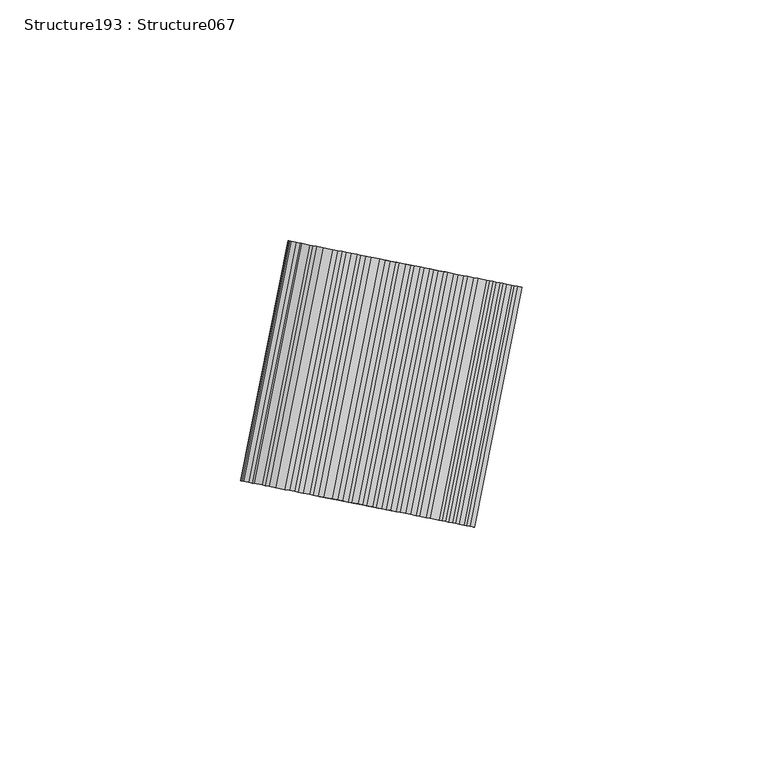
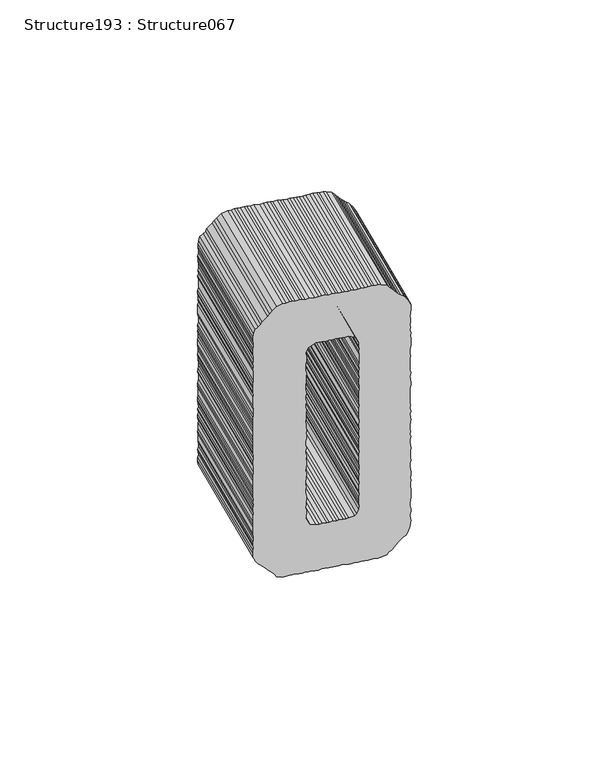
"""IFC4 building model written with IfcOpenShell, lengths in millimetres: proxy geometry, Structure193 : Structure067."""

from ifc_helpers import new_model, si_unit, frame, origin, place, context, project, spatial, polyline, outline, extrude, source, transform, mapped, element, save


def structure193_structure067_310a77a5(model_context):
    return source(origin(), model_context, "Body", "SweptSolid", [
        extrude(outline(polyline([(1.9860445, 0.0), (2.6789094, -0.7882832), (3.8239592, -1.2173664), (5.3807844, -2.3653471), (6.3497852, -3.2236496), (7.0882408, -3.6107772), (8.0066377, -4.2175769), (9.1528806, -4.65259), (9.8415639, -5.445344), (10.8594989, -7.2214925), (11.1707558, -8.0920017), (11.5266802, -9.2097639), (11.5546014, -9.9997252), (11.6286641, -11.0442649), (12.1416474, -12.266168), (12.3476425, -13.2899692), (12.2954284, -14.3581017), (12.5003006, -15.3763217), (12.8104345, -16.2412497), (13.1408113, -17.2320396), (13.7306521, -20.1635644), (13.8103704, -21.2109584), (14.040369, -22.3540577), (14.3966443, -23.4735641), (14.4256886, -24.2691066), (14.781613, -25.3868688), (14.9872571, -26.4089259), (15.0395329, -27.3199294), (15.139845, -28.4949295), (15.3454892, -29.5169867), (15.7807769, -30.3527405), (15.8859726, -31.526758), (16.3216154, -33.6919144), (16.6775398, -34.8096767), (16.7321316, -35.7321914), (16.8312506, -36.9012615), (17.0114174, -37.7966951), (17.4985021, -38.8898819), (17.4210914, -39.8327863), (17.7826715, -40.9534029), (17.8049371, -41.7405098), (18.0616063, -43.0161625), (18.7284366, -45.0026899), (18.7567089, -45.7943953), (18.8558279, -46.9634655), (19.2919578, -47.8034053), (19.2408667, -48.877119), (19.6016747, -49.9938986), (19.6764393, -51.0419265), (20.7011507, -56.1347704), (21.1636003, -57.1055196), (21.3935287, -58.2482701), (21.4218009, -59.0399755), (21.5221131, -60.2149756), (22.0339734, -61.4312976), (21.9577558, -62.3801319), (22.7775952, -66.454756), (23.138333, -67.5711868), (23.2132379, -68.6199123), (23.4180399, -69.6377835), (24.0334943, -71.368971), (24.4953163, -73.664239), (24.5743328, -74.7081449), (24.8784601, -75.5684743), (24.8021724, -76.5169599), (25.1629804, -77.6337395), (25.2126185, -78.556888), (25.5734967, -79.6740165), (25.7528914, -80.5656131), (25.8276559, -81.6136409), (26.5443883, -83.8481827), (26.9297079, -85.7632317), (26.371283, -87.5984982), (25.7853557, -88.6440823), (25.4039476, -89.3802981), (24.5409722, -90.351328), (23.9028991, -91.1395494), (23.397037, -91.9066133), (22.8107609, -92.9522675), (22.304197, -93.7158431), (21.6937749, -94.6396873), (21.2071753, -95.5295438), (19.5530517, -96.5280079), (18.6869304, -96.8322118), (17.412673, -97.0886002), (16.6774334, -97.3686475), (15.5294505, -97.5996287), (14.4863807, -97.6773882), (13.338049, -97.9084396), (12.4216748, -97.9628847), (11.2782267, -98.1929535), (10.4068731, -98.4982102), (9.4904989, -98.5526553), (8.3721773, -98.9076035), (7.5817289, -98.9367116), (6.3074714, -99.1931), (5.5669273, -99.472037), (4.5753013, -99.8036708), (3.2503698, -99.8082076), (2.535722, -100.2140467), (1.3922738, -100.4441155), (0.3443204, -100.5228576), (-0.8287889, -100.6289594), (-2.5564243, -101.2386178), (-3.7550812, -101.2177474), (-4.7219295, -101.6743307), (-5.4872513, -101.8283182), (-6.7870564, -101.9577344), (-7.7790312, -102.2894384), (-8.544353, -102.4434258), (-9.6125495, -102.396306), (-10.6349554, -102.6020203), (-12.672446, -102.3463317), (-14.3292984, -101.3524044), (-15.2483972, -100.7421164), (-16.0409385, -100.1096308), (-18.0013673, -98.911108), (-18.5634229, -98.0965052), (-19.4562021, -97.6170265), (-20.6279926, -97.0550411), (-21.3186987, -95.6010422), (-21.674623, -94.48328), (-21.9046216, -93.3401807), (-21.9842698, -92.2931354), (-22.1635943, -91.4018877), (-22.626465, -90.4290457), (-22.6749099, -89.5118271), (-22.8794311, -88.4953512), (-22.9583774, -87.4517943), (-23.189499, -86.3031137), (-23.5461954, -85.1815144), (-23.6250715, -84.1383062), (-24.0611312, -83.2987152), (-24.0101104, -82.2246527), (-24.650555, -79.0416252), (-25.0854918, -78.2076154), (-25.3166134, -77.0589349), (-25.340002, -76.2662469), (-25.59625, -74.9926871), (-25.6497189, -74.0757535), (-26.0857786, -73.2361625), (-26.7262233, -70.0531351), (-26.7258063, -68.7275697), (-27.1099328, -66.8184508), (-27.5468347, -65.974674), (-27.6715013, -64.6786316), (-27.9565789, -63.9382341), (-28.0314137, -62.8898573), (-28.2358647, -61.8737304), (-28.5727394, -60.8759), (-28.9808693, -58.847483), (-29.0556339, -57.7994551), (-29.2605761, -56.7808864), (-29.6476336, -55.5336463), (-29.6973419, -54.6101489), (-29.9017929, -53.5940218), (-29.9818622, -52.5448836), (-30.1856113, -51.5322449), (-30.5422375, -50.4109944), (-30.879042, -49.4135129), (-30.8005084, -48.4761896), (-31.1855472, -46.5625361), (-31.6722108, -45.4714423), (-31.8527285, -44.5742647), (-31.9519177, -43.4048457), (-32.4130378, -41.1130659), (-32.7231718, -40.2481378), (-32.9280439, -39.2299179), (-33.0028786, -38.1815412), (-33.1080744, -37.0075237), (-33.5430111, -36.1735138), (-33.5173975, -34.9731767), (-33.9279798, -34.2602091), (-34.1336239, -33.2381521), (-34.1072383, -32.041652), (-34.4125587, -31.1753925), (-34.8481313, -29.010585), (-35.1571423, -28.1512381), (-35.2323279, -27.1011173), (-35.6930972, -24.8110817), (-35.7731664, -23.7619435), (-35.952491, -22.8706958), (-36.4137474, -21.9058766), (-36.4622624, -20.9883093), (-36.5419808, -19.9409152), (-37.0035881, -18.9743519), (-37.2335867, -17.8312526), (-37.3338989, -16.6562525), (-36.8766221, -14.9712725), (-36.4462117, -13.8274074), (-35.8096105, -13.033675), (-35.3026977, -12.2700292), (-34.6660964, -11.4762968), (-33.9527013, -10.4112356), (-33.4723868, -9.5171994), (-32.3486946, -7.8360522), (-31.8935768, -6.8167879), (-30.2394531, -5.8183238), (-29.0648018, -5.7180817), (-28.022153, -5.6382292), (-27.1560318, -5.3340255), (-26.2393088, -5.27951), (-25.1209872, -4.924562), (-24.2248559, -4.7442549), (-22.925472, -4.6127457), (-22.1901602, -4.3348616), (-21.016702, -4.2286895), (-20.1765516, -3.7936062), (-19.1593781, -3.5889446), (-18.0855261, -3.6389189), (-17.1942784, -3.4595944), (-16.0759568, -3.1046463), (-13.0139715, -2.4885561), (-11.9762063, -2.4096862), (-10.9541492, -2.2040421), (-9.9880731, -1.7436217), (-9.0968253, -1.5642972), (-8.1740256, -1.5147293), (-7.0568972, -1.1538512), (-5.8574682, -1.1785586), (-4.9909981, -0.8742846), (-3.9734759, -0.6695529), (-2.8003666, -0.5634509), (-1.7828442, -0.3587192), (-0.916723, -0.0545154), (0.0, 0.0), (1.9860445, 0.0)]), holes=[polyline([(-6.2250852, -83.6817193), (-3.6710508, -84.4987575), (-2.6790739, -84.1688678), (-1.7622808, -84.1147013), (-0.7961344, -83.6546297), (0.2772986, -83.7043254), (1.2434449, -83.2442538), (2.3119944, -83.2949321), (3.3295167, -83.0902004), (4.4526517, -82.7339208), (5.3690961, -82.6798245), (6.391502, -82.4741101), (8.0156155, -81.3517493), (8.4004354, -80.6090398), (8.7534309, -79.0804209), (8.4971828, -77.806861), (8.549116, -76.7373333), (8.2437955, -75.8710738), (8.1385998, -74.6970562), (7.5247555, -71.6462335), (7.1130503, -70.9276846), (7.1143094, -69.6063052), (6.652632, -68.6393932), (6.6296644, -67.8487981), (6.498921, -66.5478083), (6.0620894, -65.7043802), (5.8835369, -64.8169696), (5.884024, -63.4917531), (5.7034361, -62.5942265), (5.2167726, -61.5031327), (5.1430607, -60.4603373), (4.8580534, -59.7202885), (4.809468, -58.8023724), (4.4730847, -57.8069838), (4.4998914, -56.6125767), (4.1438968, -55.4944656), (3.7589282, -53.5811609), (3.4232468, -52.5892605), (3.4488603, -51.3889234), (2.7816791, -49.4006518), (2.833893, -48.3325193), (2.4240829, -47.6233888), (2.3237706, -46.4483887), (2.2703719, -45.531804), (1.8079927, -44.5614036), (1.7339299, -43.516864), (1.4776818, -42.2433042), (1.1930254, -41.5049995), (1.2448884, -40.4351229), (0.7581547, -39.3436803), (0.734766, -38.5509923), (0.2984214, -36.3823478), (0.2194751, -35.3387907), (-0.0105235, -34.1956914), (-0.2906473, -33.4546601), (-0.3947201, -32.2862238), (-0.7251671, -31.295085), (-1.0364239, -30.4245757), (-0.9845609, -29.3546991), (-1.3412574, -28.2330997), (-1.725454, -26.3236321), (-1.8051723, -25.2762381), (-2.1610967, -24.1584758), (-2.3914462, -23.0136324), (-2.6772256, -22.2697466), (-2.6504891, -21.0749906), (-3.0064135, -19.9572284), (-3.9549755, -18.5511193), (-4.6960006, -18.1746712), (-6.5508847, -18.1500956), (-7.4688009, -18.198681), (-8.3600486, -18.3780055), (-9.4820606, -18.7398662), (-10.399628, -18.7883814), (-11.3908307, -19.1239225), (-12.6914077, -19.2495015), (-13.4822071, -19.2768656), (-14.7309871, -19.6598774), (-15.648061, -19.7126487), (-16.7442468, -20.2010627), (-18.3242416, -20.9167569), (-19.0065696, -23.4386056), (-18.8272451, -24.3298533), (-18.4713207, -25.4476155), (-18.2908031, -26.3447932), (-18.3378527, -27.4133384), (-17.9819283, -28.5311007), (-17.8017616, -29.4265343), (-17.4710339, -30.4190684), (-17.2916392, -31.3106649), (-17.2872427, -32.6348988), (-17.0823706, -33.6531187), (-16.7515727, -34.6460017), (-16.6719245, -35.6930469), (-16.4925299, -36.5846434), (-16.1359036, -37.705894), (-15.6509077, -39.4651452), (-15.6982381, -40.5322951), (-15.3423137, -41.6500574), (-15.0359404, -42.5215492), (-14.8576687, -43.4075646), (-14.7269955, -44.7082055), (-14.4209732, -45.5779533), (-14.4428262, -46.7717266), (-14.2885579, -47.5384439), (-13.8322554, -48.5038967), (-13.8792348, -49.5727908), (-13.6218638, -50.8519318), (-13.1651401, -51.8194777), (-12.9606189, -52.8359536), (-12.9323467, -53.627659), (-12.5764223, -54.7454212), (-12.4967742, -55.7924665), (-12.291902, -56.8106865), (-12.2133067, -57.8524993), (-11.8554873, -58.9796798), (-11.4724838, -60.8832175), (-11.1660403, -61.7550582), (-11.1878933, -62.9488315), (-11.0073757, -63.8460093), (-10.5773225, -64.6810016), (-10.6243722, -65.7495469), (-10.4186579, -66.7719528), (-9.9368778, -67.8640292), (-9.9576079, -69.0633837), (-9.5470916, -71.1036607), (-9.2673889, -71.8425991), (-8.8579254, -73.8776437), (-8.5260747, -74.8757591), (-8.5479277, -76.0695324), (-8.1378326, -78.1077164), (-7.6555613, -79.2022346), (-7.2969123, -80.98473), (-7.3442427, -82.0518799), (-6.2250852, -83.6817193)])]), frame((-2353.2918916, 234935.5090639, 386.7894186), z_axis=(0.19466222296394123, 0.9808703374813295, 0.0), x_axis=(0.9615988088498644, -0.19083762101609555, 0.19725296759095734)), (0.0, 0.0, 1.0), 50.8),
    ])


if __name__ == "__main__":
    model = new_model("IFC4")
    model_context = context("Model", 3, world=origin())
    ifc_project = project(units=[si_unit("LENGTHUNIT", "METRE", prefix="MILLI")], contexts=[model_context])
    site = spatial("IfcSite", under=ifc_project)
    building = spatial("IfcBuilding", under=site)
    placement = place(None, origin())
    structure193_structure067_shape = structure193_structure067_310a77a5(model_context)
    element("IfcBuildingElementProxy", 1, Name="Structure193 : Structure067", ObjectType="Structure193 : Structure067", at=placement, inside=building, context=model_context, shape_type="MappedRepresentation", body=[
        mapped(structure193_structure067_shape, transform((0.0, 0.0, 0.0), x_axis=(1.0, 0.0, 0.0), y_axis=(0.0, 1.0, 0.0), z_axis=(0.0, 0.0, 1.0))),
    ])
    save(model, "model.ifc")

# Revit data of these elements
# Type "Structure193 : Structure067"
#   NameOverride = "Structure067"
# Element 1 (IfcBuildingElementProxy, "Structure193 : Structure067")
#   Materials on its faces: "BRUSHED ALUMINUM LETTERING"
# Materials
#   "BRUSHED ALUMINUM LETTERING": class "Unassigned", colour RGB 169 181 186, transparency 0, Cost = 0
